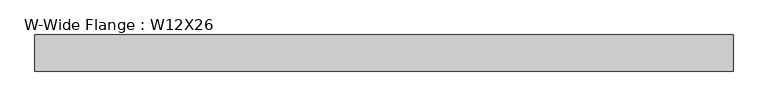
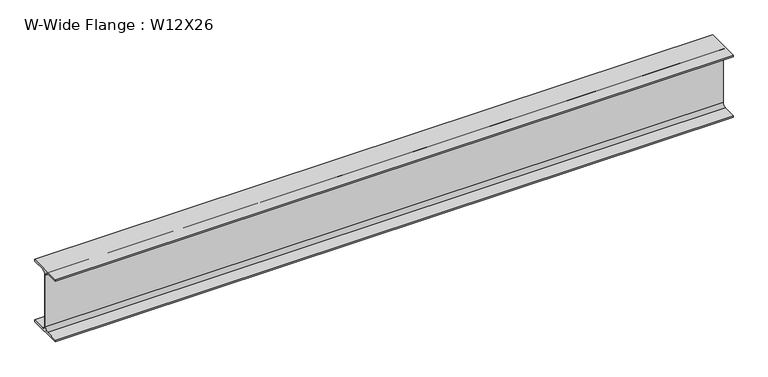
"""IFC4 building model written with IfcOpenShell, lengths in millimetres: beam geometry, W-Wide Flange : W12X26."""

from ifc_helpers import new_model, si_unit, point, frame, frame_2d, origin, place, context, project, spatial, polyline, circle_curve, trimmed, segment, composite_curve, outline, extrude, source, transform, mapped, element, save


def w_wide_flange_w12x26_4149ab62(model_context):
    return source(origin(), model_context, "Body", "SweptSolid", [
        extrude(outline(composite_curve([segment(polyline([(82.4011719, -145.5539063), (82.4011719, -155.178125), (-82.4011719, -155.178125), (-82.4011719, -145.5539063), (-20.2902344, -145.5539063)]), True, "CONTINUOUS"), segment(trimmed(circle_curve(frame_2d((-20.2902344, -128.190625)), 17.3632812), [point((-20.2902344, -145.5539063))], [point((-2.9269531, -128.190625))], True, "CARTESIAN"), True, "CONTINUOUS"), segment(polyline([(-2.9269531, -128.190625), (-2.9269531, 128.190625)]), True, "CONTINUOUS"), segment(trimmed(circle_curve(frame_2d((-20.2902344, 128.190625)), 17.3632812), [point((-2.9269531, 128.190625))], [point((-20.2902344, 145.5539062))], True, "CARTESIAN"), True, "CONTINUOUS"), segment(polyline([(-20.2902344, 145.5539062), (-82.4011719, 145.5539062), (-82.4011719, 155.178125), (82.4011719, 155.178125), (82.4011719, 145.5539062), (20.2902344, 145.5539062)]), True, "CONTINUOUS"), segment(trimmed(circle_curve(frame_2d((20.2902344, 128.190625)), 17.3632812), [point((20.2902344, 145.5539062))], [point((2.9269531, 128.190625))], True, "CARTESIAN"), True, "CONTINUOUS"), segment(polyline([(2.9269531, 128.190625), (2.9269531, -128.190625)]), True, "CONTINUOUS"), segment(trimmed(circle_curve(frame_2d((20.2902344, -128.190625)), 17.3632812), [point((2.9269531, -128.190625))], [point((20.2902344, -145.5539063))], True, "CARTESIAN"), True, "CONTINUOUS"), segment(polyline([(20.2902344, -145.5539063), (82.4011719, -145.5539063)]), True, "CONTINUOUS")], self_intersect=False)), frame((-1535.865688, 0.0, 0.0), z_axis=(1.0, 0.0, 0.0), x_axis=(0.0, 1.0, 0.0)), (0.0, 0.0, 1.0), 3186.0313761),
    ])


if __name__ == "__main__":
    model = new_model("IFC4")
    model_context = context("Model", 3, world=origin())
    ifc_project = project(units=[si_unit("LENGTHUNIT", "METRE", prefix="MILLI")], contexts=[model_context])
    site = spatial("IfcSite", under=ifc_project)
    building = spatial("IfcBuilding", under=site)
    placement = place(None, origin())
    w_wide_flange_w12x26_shape = w_wide_flange_w12x26_4149ab62(model_context)
    element("IfcBeam", 1, ObjectType="W-Wide Flange : W12X26", at=placement, inside=building, context=model_context, shape_type="MappedRepresentation", body=[
        mapped(w_wide_flange_w12x26_shape, transform((0.0, 0.0, 0.0), x_axis=(1.0, 0.0, 0.0), y_axis=(0.0, 1.0, 0.0), z_axis=(0.0, 0.0, 1.0))),
    ])
    save(model, "model.ifc")

# Revit data of these elements
# Type "W-Wide Flange : W12X26"
#   Assembly Code = "B10"
#   W = 26
#   Length [instance default] = 5' - 0"
#   bf = 0' - 6 125/256"
#   d = 1' - 0 7/32"
#   k = 0' - 1 1/16"
#   k2 = 0' - 0 175/256"
#   tf = 0' - 0 97/256"
#   tw = 0' - 0 59/256"
#   A = 0.053125 SF
#   Structural Material [instance default] = none
# Element 1 (IfcBeam, "W-Wide Flange : W12X26")
#   Structural Material = Dark metal
#   Materials on its faces: "Dark metal"
# Materials
#   "Dark metal": class "Generic", colour RGB 44 29 29, transparency 0, Cost = 0
